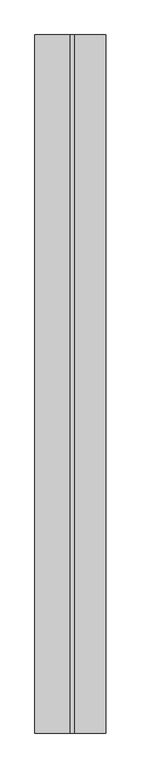
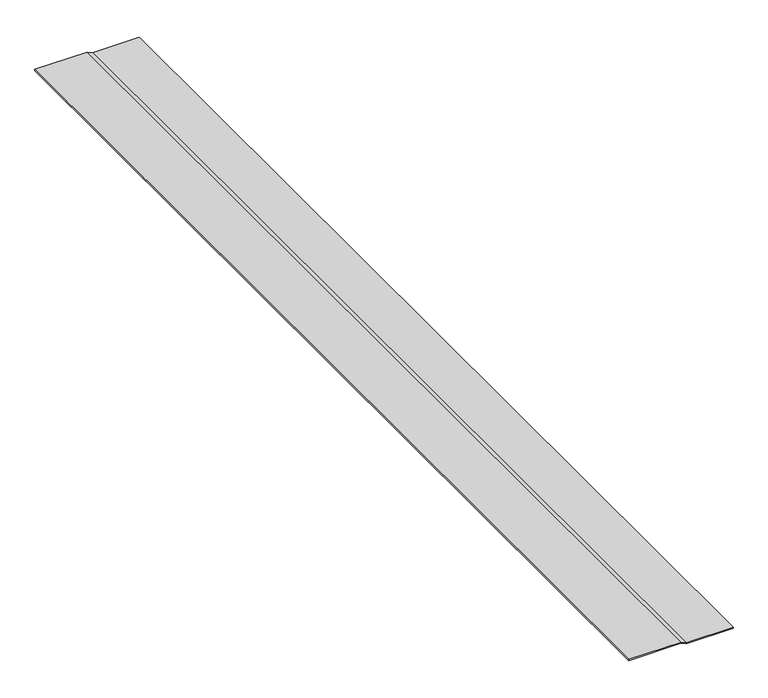
"""IFC4 building model written with IfcOpenShell, lengths in millimetres: proxy geometry, INTERPLY003 : INTERPLY003."""

from ifc_helpers import new_model, si_unit, frame, origin, place, context, project, spatial, polyline, outline, extrude, source, transform, mapped, element, save


def generic_models_3c302f4a(model_context):
    return source(origin(), model_context, "Body", "SweptSolid", [
        extrude(outline(polyline([(40265.8733085, -2677.2016654), (40265.8733085, -2778.9380547), (40263.5642176, -2778.9380547), (40263.5642176, -2677.6931567), (40258.8529944, -2667.127576), (40258.8529944, -2575.8980157), (40261.1620854, -2575.8980157), (40261.1620854, -2666.6360847), (40265.8733085, -2677.2016654)])), frame((0.0, 999.75, 0.0), z_axis=(0.0, 1.0, 0.0), x_axis=(0.0, 0.0, 1.0)), (0.0, 0.0, 1.0), 2000.25),
    ])


if __name__ == "__main__":
    model = new_model("IFC4")
    model_context = context("Model", 3, world=origin())
    ifc_project = project(units=[si_unit("LENGTHUNIT", "METRE", prefix="MILLI")], contexts=[model_context])
    site = spatial("IfcSite", under=ifc_project)
    building = spatial("IfcBuilding", under=site)
    placement = place(None, origin())
    generic_models_shape = generic_models_3c302f4a(model_context)
    element("IfcBuildingElementProxy", 1, Name="INTERPLY003 : INTERPLY003", ObjectType="INTERPLY003 : INTERPLY003", at=placement, inside=building, context=model_context, shape_type="MappedRepresentation", body=[
        mapped(generic_models_shape, transform((0.0, 0.0, 0.0), x_axis=(1.0, 0.0, 0.0), y_axis=(0.0, 1.0, 0.0), z_axis=(0.0, 0.0, 1.0))),
    ])
    save(model, "model.ifc")

# Revit data of these elements
# Type "INTERPLY003 : INTERPLY003"
#   NameOverride = "INTERPLY003"
# Element 1 (IfcBuildingElementProxy, "INTERPLY003 : INTERPLY003")
#   Materials on its faces: "INTERPLY"
# Materials
#   "INTERPLY": class "Unassigned", colour RGB 115 115 172, transparency 0
